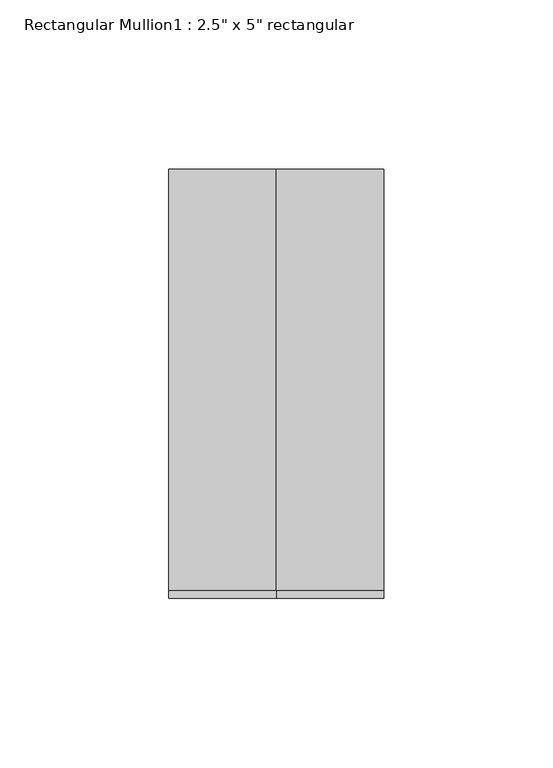
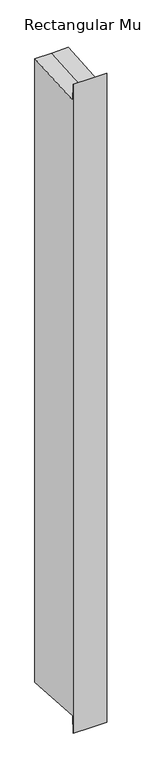
"""IFC4 building model written with IfcOpenShell, lengths in millimetres: member geometry."""

import ifcopenshell
import ifcopenshell.guid

model = None  # the IFC model being written
_history = None  # IfcOwnerHistory: only IFC2X3 demands one
_inside = {}  # id of a spatial element -> (the spatial element, [elements in it])
_under = {}  # id of a project, library or spatial element -> (it, [spatial elements below it])
_declared = {}  # id of a project -> (the project, [libraries it declares])
_typed = {}  # id of a type object -> (the type object, [elements of that type])
_made_of = {}  # id of a material, layer set ... -> (it, [elements and type objects made of it])


def new_model(schema):
    """Start an empty IFC model of exactly this schema.

    Asked for "IFC4X3", IfcOpenShell would pick the latest addendum, in which some entities
    have other attributes; the version numbers below select the first issue.
    IFC2X3 requires an IfcOwnerHistory on every rooted entity: one is made here for all.
    """
    global model, _history
    if schema == "IFC4X3":
        model = ifcopenshell.file(schema_version=(4, 3, 0, 0))
    else:
        model = ifcopenshell.file(schema=schema)
    _inside.clear()
    _under.clear()
    _declared.clear()
    _typed.clear()
    _made_of.clear()
    _history = None
    if model.schema == "IFC2X3":
        org = make("IfcOrganization", Name="unknown")
        user = make(
            "IfcPersonAndOrganization",
            ThePerson=make("IfcPerson", FamilyName="unknown"),
            TheOrganization=org,
        )
        app = make(
            "IfcApplication",
            ApplicationDeveloper=org,
            Version="unknown",
            ApplicationFullName="unknown",
            ApplicationIdentifier="unknown",
        )
        _history = make(
            "IfcOwnerHistory",
            OwningUser=user,
            OwningApplication=app,
            ChangeAction="ADDED",
            CreationDate=0,
        )
    return model


def make(cls, **values):
    """One entity of the class cls with the attributes given. An attribute that is None is left unset."""
    return model.create_entity(
        cls, **{name: value for name, value in values.items() if value is not None}
    )


def rooted(cls, **values):
    """An entity with a GlobalId (a new one), such as an element, a storey or a relation."""
    return make(cls, GlobalId=ifcopenshell.guid.new(), OwnerHistory=_history, **values)


def si_unit(unit_type, name, prefix=None):
    """IfcSIUnit, for example si_unit("LENGTHUNIT", "METRE", prefix="MILLI")."""
    return make("IfcSIUnit", UnitType=unit_type, Prefix=prefix, Name=name)


def assignment(units):
    """IfcUnitAssignment: the units of a project."""
    return None if units is None else make("IfcUnitAssignment", Units=units)


def point(xyz):
    """IfcCartesianPoint."""
    return None if xyz is None else make("IfcCartesianPoint", Coordinates=xyz)


def direction(xyz):
    """IfcDirection."""
    return None if xyz is None else make("IfcDirection", DirectionRatios=xyz)


def frame(location, z_axis=None, x_axis=None):
    """IfcAxis2Placement3D, a coordinate frame: its origin and axes. An axis left out is left unset."""
    return make(
        "IfcAxis2Placement3D",
        Location=point(location),
        Axis=direction(z_axis),
        RefDirection=direction(x_axis),
    )


def origin():
    """The frame at (0, 0, 0) with its axes left unset."""
    return frame((0.0, 0.0, 0.0))


def place(relative_to, where):
    """IfcLocalPlacement: puts the frame where relative to a parent placement (None: the world)."""
    return make(
        "IfcLocalPlacement", PlacementRelTo=relative_to, RelativePlacement=where
    )


def context(
    kind, dimensions, precision=None, world=None, true_north=None, identifier=None
):
    """IfcGeometricRepresentationContext, for example the 3D "Model" context."""
    return make(
        "IfcGeometricRepresentationContext",
        ContextIdentifier=identifier,
        ContextType=kind,
        CoordinateSpaceDimension=dimensions,
        Precision=precision,
        WorldCoordinateSystem=world,
        TrueNorth=true_north,
    )


def project(units=None, contexts=None):
    """IfcProject with its units and contexts."""
    return rooted(
        "IfcProject",
        Name="project",
        RepresentationContexts=contexts,
        UnitsInContext=assignment(units),
    )


def spatial(cls, under=None, at=None, **own):
    """A site, building, storey or space (cls), placed at a placement, below another one or the project."""
    s = rooted(cls, ObjectPlacement=at, **own)
    if under is not None:
        _under.setdefault(under.id(), (under, []))[1].append(s)
    return s


def faces_of(points, faces, orient=None, outer=None):
    """IfcFace entities. A face is a list of loops; a loop is a list of indices into points, from 0.

    orient and outer hold one flag for each loop. By default every Orientation is true, the
    first loop of a face is its IfcFaceOuterBound and the others are IfcFaceBound.
    """
    made = []
    for i, loops in enumerate(faces):
        bounds = []
        for j, loop in enumerate(loops):
            is_outer = j == 0 if outer is None else outer[i][j]
            bounds.append(
                make(
                    "IfcFaceOuterBound" if is_outer else "IfcFaceBound",
                    Bound=make("IfcPolyLoop", Polygon=[points[k] for k in loop]),
                    Orientation=True if orient is None else orient[i][j],
                )
            )
        made.append(make("IfcFace", Bounds=bounds))
    return made


def faceted_brep(points, faces, orient=None, outer=None, voids=None):
    """IfcFacetedBrep: a solid bounded by flat faces; with voids (closed shells), ...WithVoids."""
    shared = [point(p) for p in points]
    hull = make("IfcClosedShell", CfsFaces=faces_of(shared, faces, orient, outer))
    if voids is None:
        return make("IfcFacetedBrep", Outer=hull)
    return make(
        "IfcFacetedBrepWithVoids",
        Outer=hull,
        Voids=[
            make(cls, CfsFaces=faces_of(shared, fs, o, b)) for cls, fs, o, b in voids
        ],
    )


def shape(context_of_items, identifier, shape_type, items):
    """IfcShapeRepresentation: the items that make up one representation, for example the "Body"."""
    return make(
        "IfcShapeRepresentation",
        ContextOfItems=context_of_items,
        RepresentationIdentifier=identifier,
        RepresentationType=shape_type,
        Items=items,
    )


def source(mapping_origin, context_of_items, identifier, shape_type, items):
    """IfcRepresentationMap: a shape defined once, which mapped items show again and again."""
    return make(
        "IfcRepresentationMap",
        MappingOrigin=mapping_origin,
        MappedRepresentation=shape(context_of_items, identifier, shape_type, items),
    )


def transform(
    local_origin,
    x_axis=None,
    y_axis=None,
    z_axis=None,
    scale=None,
    scale2=None,
    scale3=None,
    uniform=True,
):
    """IfcCartesianTransformationOperator3D, or its non-uniform kind. x_axis, y_axis, z_axis: its Axis1, 2, 3."""
    if uniform:
        return make(
            "IfcCartesianTransformationOperator3D",
            Axis1=direction(x_axis),
            Axis2=direction(y_axis),
            LocalOrigin=point(local_origin),
            Scale=scale,
            Axis3=direction(z_axis),
        )
    return make(
        "IfcCartesianTransformationOperator3DnonUniform",
        Axis1=direction(x_axis),
        Axis2=direction(y_axis),
        LocalOrigin=point(local_origin),
        Scale=scale,
        Axis3=direction(z_axis),
        Scale2=scale2,
        Scale3=scale3,
    )


def mapped(mapping_source, mapping_target):
    """IfcMappedItem: shows the shape of a source again, moved by a transform."""
    return make(
        "IfcMappedItem", MappingSource=mapping_source, MappingTarget=mapping_target
    )


def made_of(thing, what):
    """Note that an element or type object is made of a material, layer set ...; save() writes the relation."""
    if what is not None:
        _made_of.setdefault(what.id(), (what, []))[1].append(thing)
    return thing


def element(
    cls,
    number,
    at=None,
    inside=None,
    cuts=None,
    type_object=None,
    material=None,
    context=None,
    identifier="Body",
    shape_type=None,
    held_by="IfcProductDefinitionShape",
    body=None,
    shapes=None,
    **own,
):
    """One element of the class cls, such as IfcWall. Its Tag is "e" and its number.

    at: its placement. inside: the storey or other place that contains it. cuts: it is an
    opening in that element (IfcRelVoidsElement). A single representation is given by context,
    identifier, shape_type and body (its items); several are given by shapes. held_by: the class
    of the entity that holds the representations. save() writes the other relations.
    """
    e = rooted(cls, Tag="e%d" % number, ObjectPlacement=at, **own)
    if body is not None:
        shapes = [shape(context, identifier, shape_type, body)]
    if shapes is not None:
        e.Representation = make(held_by, Representations=shapes)
    if inside is not None:
        _inside.setdefault(inside.id(), (inside, []))[1].append(e)
    if cuts is not None:
        rooted(
            "IfcRelVoidsElement", RelatingBuildingElement=cuts, RelatedOpeningElement=e
        )
    if type_object is not None:
        _typed.setdefault(type_object.id(), (type_object, []))[1].append(e)
    return made_of(e, material)


def aggregate(whole, parts):
    """IfcRelAggregates: a whole, such as a stair, and the parts it consists of."""
    return rooted("IfcRelAggregates", RelatingObject=whole, RelatedObjects=parts)


def save(model, path):
    """Write the relations noted so far, then the file.

    IfcRelAggregates (storeys below a building ...), IfcRelContainedInSpatialStructure (elements
    in a storey), IfcRelDefinesByType, IfcRelAssociatesMaterial and IfcRelDeclares: one each for
    every whole, place, type object, material and project.
    """
    for whole, parts in _under.values():
        aggregate(whole, parts)
    for where, things in _inside.values():
        rooted(
            "IfcRelContainedInSpatialStructure",
            RelatedElements=things,
            RelatingStructure=where,
        )
    for kind, things in _typed.values():
        rooted("IfcRelDefinesByType", RelatedObjects=things, RelatingType=kind)
    for what, things in _made_of.values():
        rooted("IfcRelAssociatesMaterial", RelatedObjects=things, RelatingMaterial=what)
    for by, libraries in _declared.values():
        rooted("IfcRelDeclares", RelatingContext=by, RelatedDefinitions=libraries)
    model.write(path)


def member_9c235780(model_context):
    return source(origin(), model_context, "Body", "Brep", [
        faceted_brep([(-31.75, 63.5, 4.2249441), (0.0, 63.5, 4.2249441), (31.75, 63.5, 4.2249441), (31.75, 63.5, -1253.4859011), (0.0, 63.5, -1253.4859011), (-31.75, 63.5, -1253.4859011), (-31.75, -63.5, 29.6036678), (-31.75, -61.2111885, -4.2153013), (-31.75, -61.2111885, -1245.0456557), (-31.75, -63.5, -1278.8646248), (31.75, -63.5, 29.6036678), (0.0, -63.5, 29.6036678), (0.0, -63.5, -1278.8646248), (31.75, -63.5, -1278.8646248), (31.75, -61.2111885, -4.2153013), (31.75, -61.2111885, -1245.0456557), (0.0, -61.2111885, -4.2153013), (0.0, -61.2111885, -1245.0456557)], [[[0, 1, 2, 3, 4, 5]], [[6, 7, 0, 5, 8, 9]], [[10, 11, 6, 9, 12, 13]], [[2, 14, 10, 13, 15, 3]], [[2, 1, 16, 14]], [[1, 0, 7, 16]], [[7, 6, 11, 16]], [[11, 10, 14, 16]], [[3, 15, 17, 4]], [[15, 13, 12, 17]], [[12, 9, 8, 17]], [[8, 5, 4, 17]]]),
    ])


if __name__ == "__main__":
    model = new_model("IFC4")
    model_context = context("Model", 3, world=origin())
    ifc_project = project(units=[si_unit("LENGTHUNIT", "METRE", prefix="MILLI")], contexts=[model_context])
    site = spatial("IfcSite", under=ifc_project)
    building = spatial("IfcBuilding", under=site)
    placement = place(None, origin())
    member_shape = member_9c235780(model_context)
    element("IfcMember", 1, ObjectType="Rectangular Mullion1 : 2.5\" x 5\" rectangular", at=placement, inside=building, context=model_context, shape_type="MappedRepresentation", body=[
        mapped(member_shape, transform((0.0, 0.0, 0.0), x_axis=(1.0, 0.0, 0.0), y_axis=(0.0, 1.0, 0.0), z_axis=(0.0, 0.0, 1.0))),
    ])
    save(model, "model.ifc")

# Revit data of these elements
# Type "Rectangular Mullion1 : 2.5\" x 5\" rectangular"
#   built-in parameter 1007304 = 0.416667 (stored number, unit not read)
#   built-in parameter 1007301 = 0.104167 (stored number, unit not read)
#   built-in parameter 1007300 = 0.104167 (stored number, unit not read)
# Element 1 (IfcMember, "Rectangular Mullion1 : 2.5\" x 5\" rectangular")
#   Materials on its faces: "support-frame"
# Materials
#   "support-frame": class "Unassigned", colour RGB 233 233 233, transparency 0, Cost = 0
